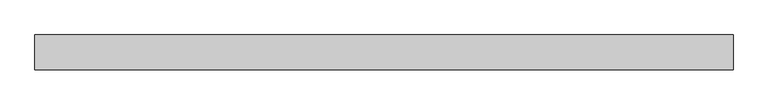
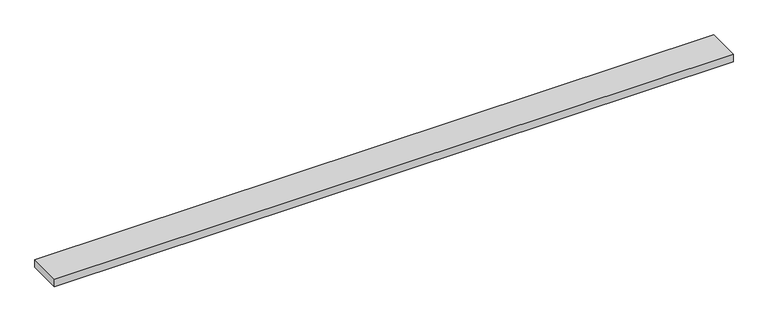
"""IFC4 building model written with IfcOpenShell, lengths in millimetres: proxy geometry, Generic Models 7:Generic Models 1:337419:Generic Models 1:337419 : Generic Models 7:Generic Models 1:337419:38 : Generic Models 7:Generic Models 1:337419:Generic Models 1:337419 : Generic Models 7:Generic Models 1:337419:301336."""

from ifc_helpers import new_model, si_unit, frame, origin, place, context, project, spatial, polyline, outline, extrude, source, transform, mapped, element, save


def generic_models_ec824403(model_context):
    return source(origin(), model_context, "Body", "SweptSolid", [
        extrude(outline(polyline([(596182.8367242, -536565.2288841), (596182.8367242, -536808.5132108), (591306.0367242, -536808.5132108), (591306.0367242, -536565.2288841), (596182.8367242, -536565.2288841)])), frame((0.0, 0.0, 8578.453125), z_axis=(0.0, 0.0, 1.0), x_axis=(1.0, 0.0, 0.0)), (0.0, 0.0, 1.0), 58.094478),
    ])


if __name__ == "__main__":
    model = new_model("IFC4")
    model_context = context("Model", 3, world=origin())
    ifc_project = project(units=[si_unit("LENGTHUNIT", "METRE", prefix="MILLI")], contexts=[model_context])
    site = spatial("IfcSite", under=ifc_project)
    building = spatial("IfcBuilding", under=site)
    placement = place(None, origin())
    generic_models_shape = generic_models_ec824403(model_context)
    element("IfcBuildingElementProxy", 1, Name="Generic Models 7:Generic Models 1:337419:Generic Models 1:337419 : Generic Models 7:Generic Models 1:337419:38 : Generic Models 7:Generic Models 1:337419:Generic Models 1:337419 : Generic Models 7:Generic Models 1:337419:301336", ObjectType="Generic Models 7:Generic Models 1:337419:Generic Models 1:337419 : Generic Models 7:Generic Models 1:337419:38 : Generic Models 7:Generic Models 1:337419:Generic Models 1:337419 : Generic Models 7:Generic Models 1:337419:301336", at=placement, inside=building, context=model_context, shape_type="MappedRepresentation", body=[
        mapped(generic_models_shape, transform((0.0, 0.0, 0.0), x_axis=(1.0, 0.0, 0.0), y_axis=(0.0, 1.0, 0.0), z_axis=(0.0, 0.0, 1.0))),
    ])
    save(model, "model.ifc")

# Revit data of these elements
# Type "Generic Models 7:Generic Models 1:337419:Generic Models 1:337419 : Generic Models 7:Generic Models 1:337419:38 : Generic Models 7:Generic Models 1:337419:Generic Models 1:337419 : Generic Models 7:Generic Models 1:337419:301336"
#   NameOverride = "Generic Models 7:Generic Models 1:337419:Generic Models 1:337419 : Generic Models 7:Generic Models 1:337419:301336"
#   ObjectTypeOverride = "Generic Models 1:337419 : Generic Models 7:Generic Models 1:337419"
#   Reference = "Generic Models 1"
#   Tag = "301336"
# Element 1 (IfcBuildingElementProxy, "Generic Models 7:Generic Models 1:337419:Generic Models 1:337419 : Generic Models 7:Generic Models 1:337419:38 : Generic Models 7:Generic Models 1:337419:Generic Models 1:337419 : Generic Models 7:Generic Models 1:337419:301336")
#   Materials on its faces: "RIGID INSULATION AT GIRTS/JAMB - (CLASS A FLAME SPREAD)"
# Materials
#   "RIGID INSULATION AT GIRTS/JAMB - (CLASS A FLAME SPREAD)": class "Unassigned", colour RGB 205 188 106, transparency 0, Cost = 0
